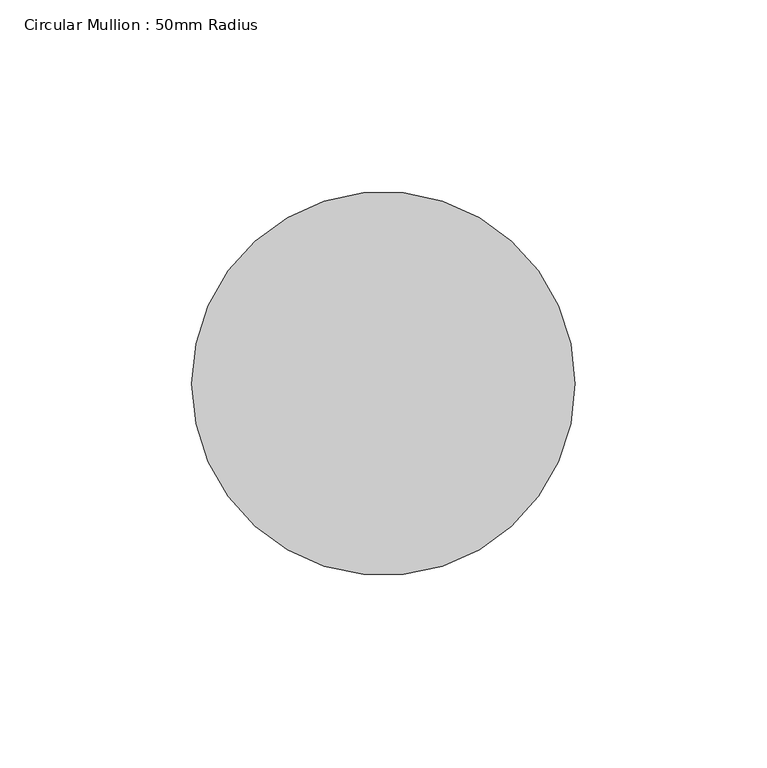
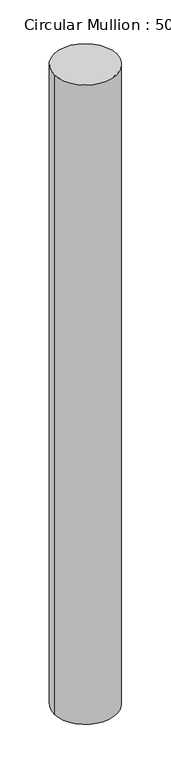
"""IFC4 building model written with IfcOpenShell, lengths in millimetres: member geometry, Circular Mullion : 50mm Radius."""

from ifc_helpers import new_model, si_unit, point, frame, origin, origin_2d, place, context, project, spatial, circle_curve, trimmed, segment, composite_curve, outline, extrude, source, transform, mapped, element, save


def circular_mullion_50mm_radius_95bae5d6(model_context):
    return source(origin(), model_context, "Body", "SweptSolid", [
        extrude(outline(composite_curve([segment(trimmed(circle_curve(origin_2d(), 50.0), [point((50.0, 0.0))], [point((-50.0, 0.0))], False, "CARTESIAN"), True, "CONTINUOUS"), segment(trimmed(circle_curve(origin_2d(), 50.0), [point((-50.0, 0.0))], [point((50.0, 0.0))], False, "CARTESIAN"), True, "CONTINUOUS")], self_intersect=False)), frame((0.0, 0.0, -1082.5234459), z_axis=(0.0, 0.0, 1.0), x_axis=(1.0, 0.0, 0.0)), (0.0, 0.0, 1.0), 1082.5234459),
    ])


if __name__ == "__main__":
    model = new_model("IFC4")
    model_context = context("Model", 3, world=origin())
    ifc_project = project(units=[si_unit("LENGTHUNIT", "METRE", prefix="MILLI")], contexts=[model_context])
    site = spatial("IfcSite", under=ifc_project)
    building = spatial("IfcBuilding", under=site)
    placement = place(None, origin())
    circular_mullion_50mm_radius_shape = circular_mullion_50mm_radius_95bae5d6(model_context)
    element("IfcMember", 1, ObjectType="Circular Mullion : 50mm Radius", at=placement, inside=building, context=model_context, shape_type="MappedRepresentation", body=[
        mapped(circular_mullion_50mm_radius_shape, transform((0.0, 0.0, 0.0), x_axis=(1.0, 0.0, 0.0), y_axis=(0.0, 1.0, 0.0), z_axis=(0.0, 0.0, 1.0))),
    ])
    save(model, "model.ifc")

# Revit data of these elements
# Type "Circular Mullion : 50mm Radius"
#   built-in parameter 1007350 = 0.164042 (stored number, unit not read)
# Element 1 (IfcMember, "Circular Mullion : 50mm Radius")
#   Materials on its faces: "Aluminium"
# Materials
#   "Aluminium": class "Metal", colour RGB 247 247 247, transparency 0, Description = "Aluminium 6061", Cost = 0
